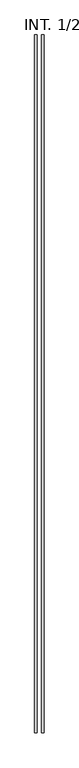
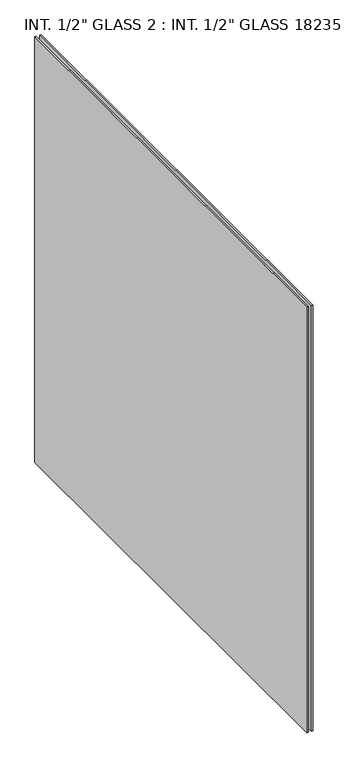
"""IFC4 building model written with IfcOpenShell, lengths in millimetres: proxy geometry."""

from ifc_helpers import new_model, si_unit, frame, origin, place, context, project, spatial, polyline, outline, extrude, source, transform, mapped, element, save


def proxy_d7a4dec2(model_context):
    return source(origin(), model_context, "Body", "SweptSolid", [
        extrude(outline(polyline([(7666.1096951, -1748.0991938), (7672.4596951, -1748.0991938), (7672.4596951, -3747.9491938), (7666.1096951, -3747.9491938), (7666.1096951, -1748.0991938)])), frame((0.0, 0.0, 37606.8963912), z_axis=(0.0, 0.0, 1.0), x_axis=(1.0, 0.0, 0.0)), (0.0, 0.0, 1.0), 1909.4026502),
        extrude(outline(polyline([(7645.9581786, -1748.0991938), (7652.3081786, -1748.0991938), (7652.3081786, -3747.9491938), (7645.9581786, -3747.9491938), (7645.9581786, -1748.0991938)])), frame((0.0, 0.0, 37606.8963912), z_axis=(0.0, 0.0, 1.0), x_axis=(1.0, 0.0, 0.0)), (0.0, 0.0, 1.0), 1909.4026502),
    ])


if __name__ == "__main__":
    model = new_model("IFC4")
    model_context = context("Model", 3, world=origin())
    ifc_project = project(units=[si_unit("LENGTHUNIT", "METRE", prefix="MILLI")], contexts=[model_context])
    site = spatial("IfcSite", under=ifc_project)
    building = spatial("IfcBuilding", under=site)
    placement = place(None, origin())
    proxy_shape = proxy_d7a4dec2(model_context)
    element("IfcBuildingElementProxy", 1, Name="INT. 1/2\" GLASS 2 : INT. 1/2\" GLASS 18235", ObjectType="INT. 1/2\" GLASS 2 : INT. 1/2\" GLASS 18235", at=placement, inside=building, context=model_context, shape_type="MappedRepresentation", body=[
        mapped(proxy_shape, transform((0.0, 0.0, 0.0), x_axis=(1.0, 0.0, 0.0), y_axis=(0.0, 1.0, 0.0), z_axis=(0.0, 0.0, 1.0))),
    ])
    save(model, "model.ifc")

# Revit data of these elements
# Type "INT. 1/2\" GLASS 2 : INT. 1/2\" GLASS 18235"
#   NameOverride = "INT. 1/2\" GLASS"
# Element 1 (IfcBuildingElementProxy, "INT. 1/2\" GLASS 2 : INT. 1/2\" GLASS 18235")
#   Materials on its faces: "1\" TEMPERED GLASS"
# Materials
#   "1\" TEMPERED GLASS": class "Unassigned", colour RGB 191 240 251, transparency 0, Cost = 0
